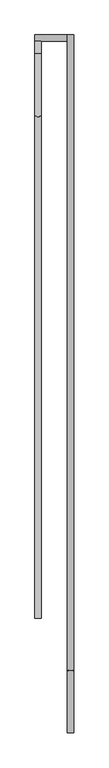
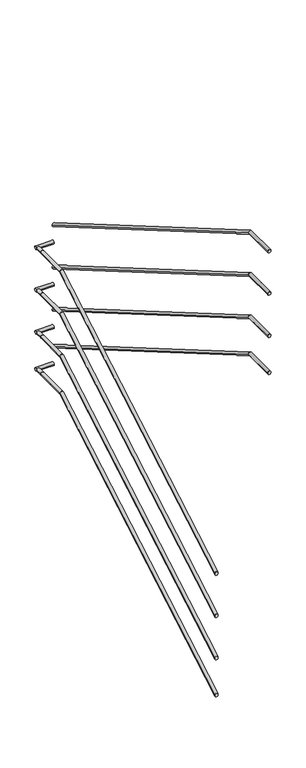
"""IFC4 building model written with IfcOpenShell, lengths in millimetres: railing geometry."""

from ifc_helpers import new_model, si_unit, frame, origin, place, context, project, spatial, circle_curve, ellipse_curve, source, transform, mapped, element, save
from ifc_brep_helpers import plane_surface, cylinder_surface, advanced_brep


def railing_7dd225d7(model_context):
    return source(origin(), model_context, "Body", "AdvancedBrep", [
        advanced_brep(
        [(52769.6, 12129.5208589, 7307.5963084), (52799.6, 12129.5208589, 7307.5963084), (52769.6, 14533.576096, 8709.9618634), (52799.6, 14533.576096, 8709.9618634), (52769.6, 14829.5208589, 8709.9618634), (52799.6, 14829.5208589, 8709.9618634)],
        [
            (0, 1, ellipse_curve(frame((52784.6, 12129.5208589, 7307.5963084), z_axis=(0.0, -1.0, 0.0), x_axis=(0.0, 0.0, -1.0)), 17.365555, 15.0)),
            (1, 0, ellipse_curve(frame((52784.6, 12129.5208589, 7307.5963084), z_axis=(0.0, -1.0, 0.0), x_axis=(0.0, 0.0, -1.0)), 17.365555, 15.0)),
            (0, 2),
            (2, 3, ellipse_curve(frame((52784.6, 14533.576096, 8709.9618634), z_axis=(0.0, -0.9653442134540491, -0.26097997921446625), x_axis=(0.0, 0.2609799792144657, -0.9653442134540494)), 15.5384989, 15.0)),
            (3, 1),
            (3, 2, ellipse_curve(frame((52784.6, 14533.576096, 8709.9618634), z_axis=(0.0, -0.9653442134540491, -0.26097997921446625), x_axis=(0.0, 0.2609799792144657, -0.9653442134540494)), 15.5384989, 15.0)),
            (4, 5, circle_curve(frame((52784.6, 14829.5208589, 8709.9618634), z_axis=(0.0, 1.0, 0.0), x_axis=(1.0, 0.0, 0.0)), 15.0)),
            (5, 4, circle_curve(frame((52784.6, 14829.5208589, 8709.9618634), z_axis=(0.0, 1.0, 0.0), x_axis=(1.0, 0.0, 0.0)), 15.0)),
            (2, 4),
            (5, 3),
        ],
        [
            plane_surface(frame((52784.6, 12129.5208589, 7324.9618634), z_axis=(0.0, -1.0, 0.0), x_axis=(0.0, 0.0, 1.0))),
            cylinder_surface(frame((52784.6, 12137.0789243, 7312.0051799), z_axis=(0.0, -0.8637789008984336, -0.5038710255240861), x_axis=(1.0, 0.0, 0.0)), 15.0),
            plane_surface(frame((52784.6, 14829.5208589, 8724.9618634), z_axis=(0.0, 1.0, 0.0), x_axis=(0.0, 0.0, 1.0))),
            cylinder_surface(frame((52784.6, 14529.5208589, 8709.9618634), z_axis=(0.0, -1.0, 0.0), x_axis=(1.0, 0.0, 0.0)), 15.0),
        ],
        [
            (0, [[1, 2]]),
            (1, [[-1, 3, 4, 5]]),
            (1, [[-2, -5, 6, -3]]),
            (2, [[7, 8]]),
            (3, [[-4, 9, -8, 10]]),
            (3, [[-6, -10, -7, -9]]),
        ],
    ),
        advanced_brep(
        [(52769.6, 14829.5208589, 8709.9618634), (52799.6, 14829.5208589, 8709.9618634), (52769.6, 14889.9208589, 8709.9618634), (52799.6, 14889.9208589, 8709.9618634)],
        [
            (0, 1, circle_curve(frame((52784.6, 14829.5208589, 8709.9618634), z_axis=(0.0, -1.0, 0.0), x_axis=(1.0, 0.0, 0.0)), 15.0)),
            (1, 0, circle_curve(frame((52784.6, 14829.5208589, 8709.9618634), z_axis=(0.0, -1.0, 0.0), x_axis=(1.0, 0.0, 0.0)), 15.0)),
            (2, 3, circle_curve(frame((52784.6, 14889.9208589, 8709.9618634), z_axis=(0.0, 1.0, 0.0), x_axis=(1.0, 0.0, 0.0)), 15.0)),
            (3, 2, circle_curve(frame((52784.6, 14889.9208589, 8709.9618634), z_axis=(0.0, 1.0, 0.0), x_axis=(1.0, 0.0, 0.0)), 15.0)),
            (0, 2),
            (3, 1),
        ],
        [
            plane_surface(frame((52784.6, 14829.5208589, 8724.9618634), z_axis=(0.0, -1.0, 0.0), x_axis=(0.0, 0.0, 1.0))),
            plane_surface(frame((52784.6, 14889.9208589, 8724.9618634), z_axis=(0.0, 1.0, 0.0), x_axis=(0.0, 0.0, 1.0))),
            cylinder_surface(frame((52784.6, 14829.5208589, 8709.9618634), z_axis=(0.0, -1.0, 0.0), x_axis=(1.0, 0.0, 0.0)), 15.0),
        ],
        [
            (0, [[1, 2]]),
            (1, [[3, 4]]),
            (2, [[-1, 5, -4, 6]]),
            (2, [[-2, -6, -3, -5]]),
        ],
    ),
        advanced_brep(
        [(52769.6, 14919.9208589, 8709.9618634), (52769.6, 14889.9208589, 8709.9618634), (52925.4, 14919.9208589, 8709.9618634), (52925.4, 14889.9208589, 8709.9618634)],
        [
            (0, 1, circle_curve(frame((52769.6, 14904.9208589, 8709.9618634), z_axis=(-1.0, 0.0, 0.0), x_axis=(0.0, -1.0, 0.0)), 15.0)),
            (1, 0, circle_curve(frame((52769.6, 14904.9208589, 8709.9618634), z_axis=(-1.0, 0.0, 0.0), x_axis=(0.0, -1.0, 0.0)), 15.0)),
            (2, 3, circle_curve(frame((52925.4, 14904.9208589, 8709.9618634), z_axis=(1.0, 0.0, 0.0), x_axis=(0.0, -1.0, 0.0)), 15.0)),
            (3, 2, circle_curve(frame((52925.4, 14904.9208589, 8709.9618634), z_axis=(1.0, 0.0, 0.0), x_axis=(0.0, -1.0, 0.0)), 15.0)),
            (0, 2),
            (3, 1),
        ],
        [
            plane_surface(frame((52769.6, 14904.9208589, 8724.9618634), z_axis=(-1.0, 0.0, 0.0), x_axis=(0.0, 1.0, 0.0))),
            plane_surface(frame((52925.4, 14904.9208589, 8724.9618634), z_axis=(1.0, 0.0, 0.0), x_axis=(0.0, 1.0, 0.0))),
            cylinder_surface(frame((52769.6, 14904.9208589, 8709.9618634), z_axis=(-1.0, 0.0, 0.0), x_axis=(0.0, -1.0, 0.0)), 15.0),
        ],
        [
            (0, [[1, 2]]),
            (1, [[3, 4]]),
            (2, [[-1, 5, -4, 6]]),
            (2, [[-2, -6, -3, -5]]),
        ],
    ),
        advanced_brep(
        [(52955.4, 14919.9208589, 8859.0296417), (52925.4, 14919.9208589, 8859.0296417), (52955.4, 11875.4656218, 10634.9618634), (52925.4, 11875.4656218, 10634.9618634), (52955.4, 11579.5208589, 10634.9618634), (52925.4, 11579.5208589, 10634.9618634)],
        [
            (0, 1, ellipse_curve(frame((52940.4, 14919.9208589, 8859.0296417), z_axis=(0.0, 1.0, 0.0), x_axis=(0.0, 0.0, -1.0)), 17.365555, 15.0)),
            (1, 0, ellipse_curve(frame((52940.4, 14919.9208589, 8859.0296417), z_axis=(0.0, 1.0, 0.0), x_axis=(0.0, 0.0, -1.0)), 17.365555, 15.0)),
            (0, 2),
            (2, 3, ellipse_curve(frame((52940.4, 11875.4656218, 10634.9618634), z_axis=(0.0, 0.9653442134540491, -0.26097997921446625), x_axis=(0.0, -0.2609799792144661, -0.9653442134540492)), 15.5384989, 15.0)),
            (3, 1),
            (3, 2, ellipse_curve(frame((52940.4, 11875.4656218, 10634.9618634), z_axis=(0.0, 0.9653442134540491, -0.26097997921446625), x_axis=(0.0, -0.2609799792144661, -0.9653442134540492)), 15.5384989, 15.0)),
            (4, 5, circle_curve(frame((52940.4, 11579.5208589, 10634.9618634), z_axis=(0.0, -1.0, 0.0), x_axis=(-1.0, 0.0, 0.0)), 15.0)),
            (5, 4, circle_curve(frame((52940.4, 11579.5208589, 10634.9618634), z_axis=(0.0, -1.0, 0.0), x_axis=(-1.0, 0.0, 0.0)), 15.0)),
            (2, 4),
            (5, 3),
        ],
        [
            plane_surface(frame((52940.4, 14919.9208589, 8876.3951967), z_axis=(0.0, 1.0, 0.0), x_axis=(0.0, 0.0, -1.0))),
            cylinder_surface(frame((52940.4, 14912.3627935, 8863.4385132), z_axis=(0.0, 0.8637789008984335, -0.5038710255240861), x_axis=(-1.0, 0.0, 0.0)), 15.0),
            plane_surface(frame((52940.4, 11579.5208589, 10649.9618634), z_axis=(0.0, -1.0, 0.0), x_axis=(0.0, 0.0, -1.0))),
            cylinder_surface(frame((52940.4, 11879.5208589, 10634.9618634), z_axis=(0.0, 1.0, 0.0), x_axis=(-1.0, 0.0, 0.0)), 15.0),
        ],
        [
            (0, [[1, 2]]),
            (1, [[-1, 3, 4, 5]]),
            (1, [[-2, -5, 6, -3]]),
            (2, [[7, 8]]),
            (3, [[-4, 9, -8, 10]]),
            (3, [[-6, -10, -7, -9]]),
        ],
    ),
        advanced_brep(
        [(52769.6, 12129.5208589, 6507.5963084), (52799.6, 12129.5208589, 6507.5963084), (52769.6, 14533.576096, 7909.9618634), (52799.6, 14533.576096, 7909.9618634), (52769.6, 14829.5208589, 7909.9618634), (52799.6, 14829.5208589, 7909.9618634)],
        [
            (0, 1, ellipse_curve(frame((52784.6, 12129.5208589, 6507.5963084), z_axis=(0.0, -1.0, 0.0), x_axis=(0.0, 0.0, -1.0)), 17.365555, 15.0)),
            (1, 0, ellipse_curve(frame((52784.6, 12129.5208589, 6507.5963084), z_axis=(0.0, -1.0, 0.0), x_axis=(0.0, 0.0, -1.0)), 17.365555, 15.0)),
            (0, 2),
            (2, 3, ellipse_curve(frame((52784.6, 14533.576096, 7909.9618634), z_axis=(0.0, -0.9653442134540491, -0.26097997921446625), x_axis=(0.0, 0.2609799792144657, -0.9653442134540494)), 15.5384989, 15.0)),
            (3, 1),
            (3, 2, ellipse_curve(frame((52784.6, 14533.576096, 7909.9618634), z_axis=(0.0, -0.9653442134540491, -0.26097997921446625), x_axis=(0.0, 0.2609799792144657, -0.9653442134540494)), 15.5384989, 15.0)),
            (4, 5, circle_curve(frame((52784.6, 14829.5208589, 7909.9618634), z_axis=(0.0, 1.0, 0.0), x_axis=(1.0, 0.0, 0.0)), 15.0)),
            (5, 4, circle_curve(frame((52784.6, 14829.5208589, 7909.9618634), z_axis=(0.0, 1.0, 0.0), x_axis=(1.0, 0.0, 0.0)), 15.0)),
            (2, 4),
            (5, 3),
        ],
        [
            plane_surface(frame((52784.6, 12129.5208589, 6524.9618634), z_axis=(0.0, -1.0, 0.0), x_axis=(0.0, 0.0, 1.0))),
            cylinder_surface(frame((52784.6, 12137.0789243, 6512.0051799), z_axis=(0.0, -0.8637789008984336, -0.5038710255240861), x_axis=(1.0, 0.0, 0.0)), 15.0),
            plane_surface(frame((52784.6, 14829.5208589, 7924.9618634), z_axis=(0.0, 1.0, 0.0), x_axis=(0.0, 0.0, 1.0))),
            cylinder_surface(frame((52784.6, 14529.5208589, 7909.9618634), z_axis=(0.0, -1.0, 0.0), x_axis=(1.0, 0.0, 0.0)), 15.0),
        ],
        [
            (0, [[1, 2]]),
            (1, [[-1, 3, 4, 5]]),
            (1, [[-2, -5, 6, -3]]),
            (2, [[7, 8]]),
            (3, [[-4, 9, -8, 10]]),
            (3, [[-6, -10, -7, -9]]),
        ],
    ),
        advanced_brep(
        [(52769.6, 14829.5208589, 7909.9618634), (52799.6, 14829.5208589, 7909.9618634), (52769.6, 14889.9208589, 7909.9618634), (52799.6, 14889.9208589, 7909.9618634)],
        [
            (0, 1, circle_curve(frame((52784.6, 14829.5208589, 7909.9618634), z_axis=(0.0, -1.0, 0.0), x_axis=(1.0, 0.0, 0.0)), 15.0)),
            (1, 0, circle_curve(frame((52784.6, 14829.5208589, 7909.9618634), z_axis=(0.0, -1.0, 0.0), x_axis=(1.0, 0.0, 0.0)), 15.0)),
            (2, 3, circle_curve(frame((52784.6, 14889.9208589, 7909.9618634), z_axis=(0.0, 1.0, 0.0), x_axis=(1.0, 0.0, 0.0)), 15.0)),
            (3, 2, circle_curve(frame((52784.6, 14889.9208589, 7909.9618634), z_axis=(0.0, 1.0, 0.0), x_axis=(1.0, 0.0, 0.0)), 15.0)),
            (0, 2),
            (3, 1),
        ],
        [
            plane_surface(frame((52784.6, 14829.5208589, 7924.9618634), z_axis=(0.0, -1.0, 0.0), x_axis=(0.0, 0.0, 1.0))),
            plane_surface(frame((52784.6, 14889.9208589, 7924.9618634), z_axis=(0.0, 1.0, 0.0), x_axis=(0.0, 0.0, 1.0))),
            cylinder_surface(frame((52784.6, 14829.5208589, 7909.9618634), z_axis=(0.0, -1.0, 0.0), x_axis=(1.0, 0.0, 0.0)), 15.0),
        ],
        [
            (0, [[1, 2]]),
            (1, [[3, 4]]),
            (2, [[-1, 5, -4, 6]]),
            (2, [[-2, -6, -3, -5]]),
        ],
    ),
        advanced_brep(
        [(52769.6, 14919.9208589, 7909.9618634), (52769.6, 14889.9208589, 7909.9618634), (52925.4, 14919.9208589, 7909.9618634), (52925.4, 14889.9208589, 7909.9618634)],
        [
            (0, 1, circle_curve(frame((52769.6, 14904.9208589, 7909.9618634), z_axis=(-1.0, 0.0, 0.0), x_axis=(0.0, -1.0, 0.0)), 15.0)),
            (1, 0, circle_curve(frame((52769.6, 14904.9208589, 7909.9618634), z_axis=(-1.0, 0.0, 0.0), x_axis=(0.0, -1.0, 0.0)), 15.0)),
            (2, 3, circle_curve(frame((52925.4, 14904.9208589, 7909.9618634), z_axis=(1.0, 0.0, 0.0), x_axis=(0.0, -1.0, 0.0)), 15.0)),
            (3, 2, circle_curve(frame((52925.4, 14904.9208589, 7909.9618634), z_axis=(1.0, 0.0, 0.0), x_axis=(0.0, -1.0, 0.0)), 15.0)),
            (0, 2),
            (3, 1),
        ],
        [
            plane_surface(frame((52769.6, 14904.9208589, 7924.9618634), z_axis=(-1.0, 0.0, 0.0), x_axis=(0.0, 1.0, 0.0))),
            plane_surface(frame((52925.4, 14904.9208589, 7924.9618634), z_axis=(1.0, 0.0, 0.0), x_axis=(0.0, 1.0, 0.0))),
            cylinder_surface(frame((52769.6, 14904.9208589, 7909.9618634), z_axis=(-1.0, 0.0, 0.0), x_axis=(0.0, -1.0, 0.0)), 15.0),
        ],
        [
            (0, [[1, 2]]),
            (1, [[3, 4]]),
            (2, [[-1, 5, -4, 6]]),
            (2, [[-2, -6, -3, -5]]),
        ],
    ),
        advanced_brep(
        [(52955.4, 14919.9208589, 8059.0296417), (52925.4, 14919.9208589, 8059.0296417), (52955.4, 11875.4656218, 9834.9618634), (52925.4, 11875.4656218, 9834.9618634), (52955.4, 11579.5208589, 9834.9618634), (52925.4, 11579.5208589, 9834.9618634)],
        [
            (0, 1, ellipse_curve(frame((52940.4, 14919.9208589, 8059.0296417), z_axis=(0.0, 1.0, 0.0), x_axis=(0.0, 0.0, -1.0)), 17.365555, 15.0)),
            (1, 0, ellipse_curve(frame((52940.4, 14919.9208589, 8059.0296417), z_axis=(0.0, 1.0, 0.0), x_axis=(0.0, 0.0, -1.0)), 17.365555, 15.0)),
            (0, 2),
            (2, 3, ellipse_curve(frame((52940.4, 11875.4656218, 9834.9618634), z_axis=(0.0, 0.9653442134540491, -0.26097997921446625), x_axis=(0.0, -0.2609799792144661, -0.9653442134540492)), 15.5384989, 15.0)),
            (3, 1),
            (3, 2, ellipse_curve(frame((52940.4, 11875.4656218, 9834.9618634), z_axis=(0.0, 0.9653442134540491, -0.26097997921446625), x_axis=(0.0, -0.2609799792144661, -0.9653442134540492)), 15.5384989, 15.0)),
            (4, 5, circle_curve(frame((52940.4, 11579.5208589, 9834.9618634), z_axis=(0.0, -1.0, 0.0), x_axis=(-1.0, 0.0, 0.0)), 15.0)),
            (5, 4, circle_curve(frame((52940.4, 11579.5208589, 9834.9618634), z_axis=(0.0, -1.0, 0.0), x_axis=(-1.0, 0.0, 0.0)), 15.0)),
            (2, 4),
            (5, 3),
        ],
        [
            plane_surface(frame((52940.4, 14919.9208589, 8076.3951967), z_axis=(0.0, 1.0, 0.0), x_axis=(0.0, 0.0, -1.0))),
            cylinder_surface(frame((52940.4, 14912.3627935, 8063.4385132), z_axis=(0.0, 0.8637789008984335, -0.5038710255240861), x_axis=(-1.0, 0.0, 0.0)), 15.0),
            plane_surface(frame((52940.4, 11579.5208589, 9849.9618634), z_axis=(0.0, -1.0, 0.0), x_axis=(0.0, 0.0, -1.0))),
            cylinder_surface(frame((52940.4, 11879.5208589, 9834.9618634), z_axis=(0.0, 1.0, 0.0), x_axis=(-1.0, 0.0, 0.0)), 15.0),
        ],
        [
            (0, [[1, 2]]),
            (1, [[-1, 3, 4, 5]]),
            (1, [[-2, -5, 6, -3]]),
            (2, [[7, 8]]),
            (3, [[-4, 9, -8, 10]]),
            (3, [[-6, -10, -7, -9]]),
        ],
    ),
        advanced_brep(
        [(52769.6, 12129.5208589, 6907.5963084), (52799.6, 12129.5208589, 6907.5963084), (52769.6, 14533.576096, 8309.9618634), (52799.6, 14533.576096, 8309.9618634), (52769.6, 14829.5208589, 8309.9618634), (52799.6, 14829.5208589, 8309.9618634)],
        [
            (0, 1, ellipse_curve(frame((52784.6, 12129.5208589, 6907.5963084), z_axis=(0.0, -1.0, 0.0), x_axis=(0.0, 0.0, -1.0)), 17.365555, 15.0)),
            (1, 0, ellipse_curve(frame((52784.6, 12129.5208589, 6907.5963084), z_axis=(0.0, -1.0, 0.0), x_axis=(0.0, 0.0, -1.0)), 17.365555, 15.0)),
            (0, 2),
            (2, 3, ellipse_curve(frame((52784.6, 14533.576096, 8309.9618634), z_axis=(0.0, -0.9653442134540491, -0.26097997921446625), x_axis=(0.0, 0.2609799792144657, -0.9653442134540494)), 15.5384989, 15.0)),
            (3, 1),
            (3, 2, ellipse_curve(frame((52784.6, 14533.576096, 8309.9618634), z_axis=(0.0, -0.9653442134540491, -0.26097997921446625), x_axis=(0.0, 0.2609799792144657, -0.9653442134540494)), 15.5384989, 15.0)),
            (4, 5, circle_curve(frame((52784.6, 14829.5208589, 8309.9618634), z_axis=(0.0, 1.0, 0.0), x_axis=(1.0, 0.0, 0.0)), 15.0)),
            (5, 4, circle_curve(frame((52784.6, 14829.5208589, 8309.9618634), z_axis=(0.0, 1.0, 0.0), x_axis=(1.0, 0.0, 0.0)), 15.0)),
            (2, 4),
            (5, 3),
        ],
        [
            plane_surface(frame((52784.6, 12129.5208589, 6924.9618634), z_axis=(0.0, -1.0, 0.0), x_axis=(0.0, 0.0, 1.0))),
            cylinder_surface(frame((52784.6, 12137.0789243, 6912.0051799), z_axis=(0.0, -0.8637789008984336, -0.5038710255240861), x_axis=(1.0, 0.0, 0.0)), 15.0),
            plane_surface(frame((52784.6, 14829.5208589, 8324.9618634), z_axis=(0.0, 1.0, 0.0), x_axis=(0.0, 0.0, 1.0))),
            cylinder_surface(frame((52784.6, 14529.5208589, 8309.9618634), z_axis=(0.0, -1.0, 0.0), x_axis=(1.0, 0.0, 0.0)), 15.0),
        ],
        [
            (0, [[1, 2]]),
            (1, [[-1, 3, 4, 5]]),
            (1, [[-2, -5, 6, -3]]),
            (2, [[7, 8]]),
            (3, [[-4, 9, -8, 10]]),
            (3, [[-6, -10, -7, -9]]),
        ],
    ),
        advanced_brep(
        [(52769.6, 14829.5208589, 8309.9618634), (52799.6, 14829.5208589, 8309.9618634), (52769.6, 14889.9208589, 8309.9618634), (52799.6, 14889.9208589, 8309.9618634)],
        [
            (0, 1, circle_curve(frame((52784.6, 14829.5208589, 8309.9618634), z_axis=(0.0, -1.0, 0.0), x_axis=(1.0, 0.0, 0.0)), 15.0)),
            (1, 0, circle_curve(frame((52784.6, 14829.5208589, 8309.9618634), z_axis=(0.0, -1.0, 0.0), x_axis=(1.0, 0.0, 0.0)), 15.0)),
            (2, 3, circle_curve(frame((52784.6, 14889.9208589, 8309.9618634), z_axis=(0.0, 1.0, 0.0), x_axis=(1.0, 0.0, 0.0)), 15.0)),
            (3, 2, circle_curve(frame((52784.6, 14889.9208589, 8309.9618634), z_axis=(0.0, 1.0, 0.0), x_axis=(1.0, 0.0, 0.0)), 15.0)),
            (0, 2),
            (3, 1),
        ],
        [
            plane_surface(frame((52784.6, 14829.5208589, 8324.9618634), z_axis=(0.0, -1.0, 0.0), x_axis=(0.0, 0.0, 1.0))),
            plane_surface(frame((52784.6, 14889.9208589, 8324.9618634), z_axis=(0.0, 1.0, 0.0), x_axis=(0.0, 0.0, 1.0))),
            cylinder_surface(frame((52784.6, 14829.5208589, 8309.9618634), z_axis=(0.0, -1.0, 0.0), x_axis=(1.0, 0.0, 0.0)), 15.0),
        ],
        [
            (0, [[1, 2]]),
            (1, [[3, 4]]),
            (2, [[-1, 5, -4, 6]]),
            (2, [[-2, -6, -3, -5]]),
        ],
    ),
        advanced_brep(
        [(52769.6, 14919.9208589, 8309.9618634), (52769.6, 14889.9208589, 8309.9618634), (52925.4, 14919.9208589, 8309.9618634), (52925.4, 14889.9208589, 8309.9618634)],
        [
            (0, 1, circle_curve(frame((52769.6, 14904.9208589, 8309.9618634), z_axis=(-1.0, 0.0, 0.0), x_axis=(0.0, -1.0, 0.0)), 15.0)),
            (1, 0, circle_curve(frame((52769.6, 14904.9208589, 8309.9618634), z_axis=(-1.0, 0.0, 0.0), x_axis=(0.0, -1.0, 0.0)), 15.0)),
            (2, 3, circle_curve(frame((52925.4, 14904.9208589, 8309.9618634), z_axis=(1.0, 0.0, 0.0), x_axis=(0.0, -1.0, 0.0)), 15.0)),
            (3, 2, circle_curve(frame((52925.4, 14904.9208589, 8309.9618634), z_axis=(1.0, 0.0, 0.0), x_axis=(0.0, -1.0, 0.0)), 15.0)),
            (0, 2),
            (3, 1),
        ],
        [
            plane_surface(frame((52769.6, 14904.9208589, 8324.9618634), z_axis=(-1.0, 0.0, 0.0), x_axis=(0.0, 1.0, 0.0))),
            plane_surface(frame((52925.4, 14904.9208589, 8324.9618634), z_axis=(1.0, 0.0, 0.0), x_axis=(0.0, 1.0, 0.0))),
            cylinder_surface(frame((52769.6, 14904.9208589, 8309.9618634), z_axis=(-1.0, 0.0, 0.0), x_axis=(0.0, -1.0, 0.0)), 15.0),
        ],
        [
            (0, [[1, 2]]),
            (1, [[3, 4]]),
            (2, [[-1, 5, -4, 6]]),
            (2, [[-2, -6, -3, -5]]),
        ],
    ),
        advanced_brep(
        [(52955.4, 14919.9208589, 8459.0296417), (52925.4, 14919.9208589, 8459.0296417), (52955.4, 11875.4656218, 10234.9618634), (52925.4, 11875.4656218, 10234.9618634), (52955.4, 11579.5208589, 10234.9618634), (52925.4, 11579.5208589, 10234.9618634)],
        [
            (0, 1, ellipse_curve(frame((52940.4, 14919.9208589, 8459.0296417), z_axis=(0.0, 1.0, 0.0), x_axis=(0.0, 0.0, -1.0)), 17.365555, 15.0)),
            (1, 0, ellipse_curve(frame((52940.4, 14919.9208589, 8459.0296417), z_axis=(0.0, 1.0, 0.0), x_axis=(0.0, 0.0, -1.0)), 17.365555, 15.0)),
            (0, 2),
            (2, 3, ellipse_curve(frame((52940.4, 11875.4656218, 10234.9618634), z_axis=(0.0, 0.9653442134540491, -0.26097997921446625), x_axis=(0.0, -0.2609799792144661, -0.9653442134540492)), 15.5384989, 15.0)),
            (3, 1),
            (3, 2, ellipse_curve(frame((52940.4, 11875.4656218, 10234.9618634), z_axis=(0.0, 0.9653442134540491, -0.26097997921446625), x_axis=(0.0, -0.2609799792144661, -0.9653442134540492)), 15.5384989, 15.0)),
            (4, 5, circle_curve(frame((52940.4, 11579.5208589, 10234.9618634), z_axis=(0.0, -1.0, 0.0), x_axis=(-1.0, 0.0, 0.0)), 15.0)),
            (5, 4, circle_curve(frame((52940.4, 11579.5208589, 10234.9618634), z_axis=(0.0, -1.0, 0.0), x_axis=(-1.0, 0.0, 0.0)), 15.0)),
            (2, 4),
            (5, 3),
        ],
        [
            plane_surface(frame((52940.4, 14919.9208589, 8476.3951967), z_axis=(0.0, 1.0, 0.0), x_axis=(0.0, 0.0, -1.0))),
            cylinder_surface(frame((52940.4, 14912.3627935, 8463.4385132), z_axis=(0.0, 0.8637789008984335, -0.5038710255240861), x_axis=(-1.0, 0.0, 0.0)), 15.0),
            plane_surface(frame((52940.4, 11579.5208589, 10249.9618634), z_axis=(0.0, -1.0, 0.0), x_axis=(0.0, 0.0, -1.0))),
            cylinder_surface(frame((52940.4, 11879.5208589, 10234.9618634), z_axis=(0.0, 1.0, 0.0), x_axis=(-1.0, 0.0, 0.0)), 15.0),
        ],
        [
            (0, [[1, 2]]),
            (1, [[-1, 3, 4, 5]]),
            (1, [[-2, -5, 6, -3]]),
            (2, [[7, 8]]),
            (3, [[-4, 9, -8, 10]]),
            (3, [[-6, -10, -7, -9]]),
        ],
    ),
        advanced_brep(
        [(52769.6, 12129.5208589, 6157.5963084), (52799.6, 12129.5208589, 6157.5963084), (52769.6, 14533.576096, 7559.9618634), (52799.6, 14533.576096, 7559.9618634), (52769.6, 14829.5208589, 7559.9618634), (52799.6, 14829.5208589, 7559.9618634)],
        [
            (0, 1, ellipse_curve(frame((52784.6, 12129.5208589, 6157.5963084), z_axis=(0.0, -1.0, 0.0), x_axis=(0.0, 0.0, -1.0)), 17.365555, 15.0)),
            (1, 0, ellipse_curve(frame((52784.6, 12129.5208589, 6157.5963084), z_axis=(0.0, -1.0, 0.0), x_axis=(0.0, 0.0, -1.0)), 17.365555, 15.0)),
            (0, 2),
            (2, 3, ellipse_curve(frame((52784.6, 14533.576096, 7559.9618634), z_axis=(0.0, -0.9653442134540491, -0.26097997921446625), x_axis=(0.0, 0.2609799792144657, -0.9653442134540494)), 15.5384989, 15.0)),
            (3, 1),
            (3, 2, ellipse_curve(frame((52784.6, 14533.576096, 7559.9618634), z_axis=(0.0, -0.9653442134540491, -0.26097997921446625), x_axis=(0.0, 0.2609799792144657, -0.9653442134540494)), 15.5384989, 15.0)),
            (4, 5, circle_curve(frame((52784.6, 14829.5208589, 7559.9618634), z_axis=(0.0, 1.0, 0.0), x_axis=(1.0, 0.0, 0.0)), 15.0)),
            (5, 4, circle_curve(frame((52784.6, 14829.5208589, 7559.9618634), z_axis=(0.0, 1.0, 0.0), x_axis=(1.0, 0.0, 0.0)), 15.0)),
            (2, 4),
            (5, 3),
        ],
        [
            plane_surface(frame((52784.6, 12129.5208589, 6174.9618634), z_axis=(0.0, -1.0, 0.0), x_axis=(0.0, 0.0, 1.0))),
            cylinder_surface(frame((52784.6, 12137.0789243, 6162.0051799), z_axis=(0.0, -0.8637789008984336, -0.5038710255240861), x_axis=(1.0, 0.0, 0.0)), 15.0),
            plane_surface(frame((52784.6, 14829.5208589, 7574.9618634), z_axis=(0.0, 1.0, 0.0), x_axis=(0.0, 0.0, 1.0))),
            cylinder_surface(frame((52784.6, 14529.5208589, 7559.9618634), z_axis=(0.0, -1.0, 0.0), x_axis=(1.0, 0.0, 0.0)), 15.0),
        ],
        [
            (0, [[1, 2]]),
            (1, [[-1, 3, 4, 5]]),
            (1, [[-2, -5, 6, -3]]),
            (2, [[7, 8]]),
            (3, [[-4, 9, -8, 10]]),
            (3, [[-6, -10, -7, -9]]),
        ],
    ),
        advanced_brep(
        [(52769.6, 14829.5208589, 7559.9618634), (52799.6, 14829.5208589, 7559.9618634), (52769.6, 14889.9208589, 7559.9618634), (52799.6, 14889.9208589, 7559.9618634)],
        [
            (0, 1, circle_curve(frame((52784.6, 14829.5208589, 7559.9618634), z_axis=(0.0, -1.0, 0.0), x_axis=(1.0, 0.0, 0.0)), 15.0)),
            (1, 0, circle_curve(frame((52784.6, 14829.5208589, 7559.9618634), z_axis=(0.0, -1.0, 0.0), x_axis=(1.0, 0.0, 0.0)), 15.0)),
            (2, 3, circle_curve(frame((52784.6, 14889.9208589, 7559.9618634), z_axis=(0.0, 1.0, 0.0), x_axis=(1.0, 0.0, 0.0)), 15.0)),
            (3, 2, circle_curve(frame((52784.6, 14889.9208589, 7559.9618634), z_axis=(0.0, 1.0, 0.0), x_axis=(1.0, 0.0, 0.0)), 15.0)),
            (0, 2),
            (3, 1),
        ],
        [
            plane_surface(frame((52784.6, 14829.5208589, 7574.9618634), z_axis=(0.0, -1.0, 0.0), x_axis=(0.0, 0.0, 1.0))),
            plane_surface(frame((52784.6, 14889.9208589, 7574.9618634), z_axis=(0.0, 1.0, 0.0), x_axis=(0.0, 0.0, 1.0))),
            cylinder_surface(frame((52784.6, 14829.5208589, 7559.9618634), z_axis=(0.0, -1.0, 0.0), x_axis=(1.0, 0.0, 0.0)), 15.0),
        ],
        [
            (0, [[1, 2]]),
            (1, [[3, 4]]),
            (2, [[-1, 5, -4, 6]]),
            (2, [[-2, -6, -3, -5]]),
        ],
    ),
        advanced_brep(
        [(52769.6, 14919.9208589, 7559.9618634), (52769.6, 14889.9208589, 7559.9618634), (52925.4, 14919.9208589, 7559.9618634), (52925.4, 14889.9208589, 7559.9618634)],
        [
            (0, 1, circle_curve(frame((52769.6, 14904.9208589, 7559.9618634), z_axis=(-1.0, 0.0, 0.0), x_axis=(0.0, -1.0, 0.0)), 15.0)),
            (1, 0, circle_curve(frame((52769.6, 14904.9208589, 7559.9618634), z_axis=(-1.0, 0.0, 0.0), x_axis=(0.0, -1.0, 0.0)), 15.0)),
            (2, 3, circle_curve(frame((52925.4, 14904.9208589, 7559.9618634), z_axis=(1.0, 0.0, 0.0), x_axis=(0.0, -1.0, 0.0)), 15.0)),
            (3, 2, circle_curve(frame((52925.4, 14904.9208589, 7559.9618634), z_axis=(1.0, 0.0, 0.0), x_axis=(0.0, -1.0, 0.0)), 15.0)),
            (0, 2),
            (3, 1),
        ],
        [
            plane_surface(frame((52769.6, 14904.9208589, 7574.9618634), z_axis=(-1.0, 0.0, 0.0), x_axis=(0.0, 1.0, 0.0))),
            plane_surface(frame((52925.4, 14904.9208589, 7574.9618634), z_axis=(1.0, 0.0, 0.0), x_axis=(0.0, 1.0, 0.0))),
            cylinder_surface(frame((52769.6, 14904.9208589, 7559.9618634), z_axis=(-1.0, 0.0, 0.0), x_axis=(0.0, -1.0, 0.0)), 15.0),
        ],
        [
            (0, [[1, 2]]),
            (1, [[3, 4]]),
            (2, [[-1, 5, -4, 6]]),
            (2, [[-2, -6, -3, -5]]),
        ],
    ),
        advanced_brep(
        [(52955.4, 14919.9208589, 7709.0296417), (52925.4, 14919.9208589, 7709.0296417), (52955.4, 11875.4656218, 9484.9618634), (52925.4, 11875.4656218, 9484.9618634), (52955.4, 11579.5208589, 9484.9618634), (52925.4, 11579.5208589, 9484.9618634)],
        [
            (0, 1, ellipse_curve(frame((52940.4, 14919.9208589, 7709.0296417), z_axis=(0.0, 1.0, 0.0), x_axis=(0.0, 0.0, -1.0)), 17.365555, 15.0)),
            (1, 0, ellipse_curve(frame((52940.4, 14919.9208589, 7709.0296417), z_axis=(0.0, 1.0, 0.0), x_axis=(0.0, 0.0, -1.0)), 17.365555, 15.0)),
            (0, 2),
            (2, 3, ellipse_curve(frame((52940.4, 11875.4656218, 9484.9618634), z_axis=(0.0, 0.9653442134540491, -0.26097997921446625), x_axis=(0.0, -0.2609799792144661, -0.9653442134540492)), 15.5384989, 15.0)),
            (3, 1),
            (3, 2, ellipse_curve(frame((52940.4, 11875.4656218, 9484.9618634), z_axis=(0.0, 0.9653442134540491, -0.26097997921446625), x_axis=(0.0, -0.2609799792144661, -0.9653442134540492)), 15.5384989, 15.0)),
            (4, 5, circle_curve(frame((52940.4, 11579.5208589, 9484.9618634), z_axis=(0.0, -1.0, 0.0), x_axis=(-1.0, 0.0, 0.0)), 15.0)),
            (5, 4, circle_curve(frame((52940.4, 11579.5208589, 9484.9618634), z_axis=(0.0, -1.0, 0.0), x_axis=(-1.0, 0.0, 0.0)), 15.0)),
            (2, 4),
            (5, 3),
        ],
        [
            plane_surface(frame((52940.4, 14919.9208589, 7726.3951967), z_axis=(0.0, 1.0, 0.0), x_axis=(0.0, 0.0, -1.0))),
            cylinder_surface(frame((52940.4, 14912.3627935, 7713.4385132), z_axis=(0.0, 0.8637789008984335, -0.5038710255240861), x_axis=(-1.0, 0.0, 0.0)), 15.0),
            plane_surface(frame((52940.4, 11579.5208589, 9499.9618634), z_axis=(0.0, -1.0, 0.0), x_axis=(0.0, 0.0, -1.0))),
            cylinder_surface(frame((52940.4, 11879.5208589, 9484.9618634), z_axis=(0.0, 1.0, 0.0), x_axis=(-1.0, 0.0, 0.0)), 15.0),
        ],
        [
            (0, [[1, 2]]),
            (1, [[-1, 3, 4, 5]]),
            (1, [[-2, -5, 6, -3]]),
            (2, [[7, 8]]),
            (3, [[-4, 9, -8, 10]]),
            (3, [[-6, -10, -7, -9]]),
        ],
    ),
    ])


if __name__ == "__main__":
    model = new_model("IFC4")
    model_context = context("Model", 3, world=origin())
    ifc_project = project(units=[si_unit("LENGTHUNIT", "METRE", prefix="MILLI")], contexts=[model_context])
    site = spatial("IfcSite", under=ifc_project)
    building = spatial("IfcBuilding", under=site)
    placement = place(None, origin())
    railing_shape = railing_7dd225d7(model_context)
    element("IfcRailing", 1, at=placement, inside=building, context=model_context, shape_type="MappedRepresentation", body=[
        mapped(railing_shape, transform((0.0, 0.0, 0.0), x_axis=(1.0, 0.0, 0.0), y_axis=(0.0, 1.0, 0.0), z_axis=(0.0, 0.0, 1.0))),
    ])
    save(model, "model.ifc")
